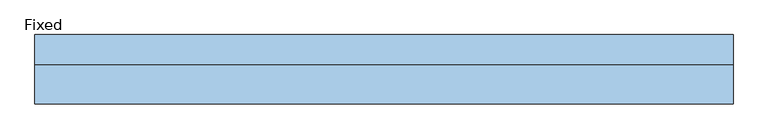
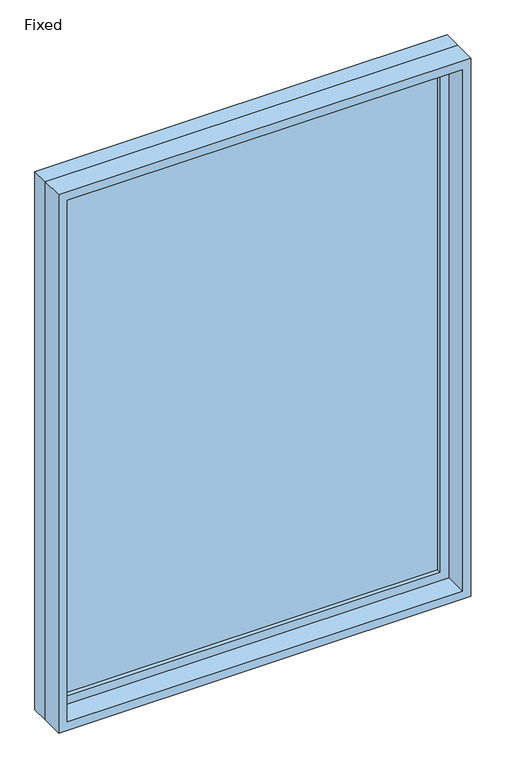
"""IFC4 building model written with IfcOpenShell, lengths in millimetres: window geometry, Fixed."""

from ifc_helpers import new_model, si_unit, frame, origin, place, context, project, spatial, polyline, outline, extrude, source, transform, mapped, element, save


def fixed_17e7873a(model_context):
    return source(origin(), model_context, "Body", "SweptSolid", [
        extrude(outline(polyline([(635.0, 25.4), (-711.2, 25.4), (-711.2, 38.1), (635.0, 38.1), (635.0, 25.4)])), frame((0.0, 0.0, 977.9), z_axis=(0.0, 0.0, 1.0), x_axis=(1.0, 0.0, 0.0)), (0.0, 0.0, 1.0), 1905.0),
        extrude(outline(polyline([(2927.35, -755.65), (933.45, -755.65), (933.45, 679.45), (2927.35, 679.45), (2927.35, -755.65)]), holes=[polyline([(2882.9, -711.2), (2882.9, 635.0), (977.9, 635.0), (977.9, -711.2), (2882.9, -711.2)])]), frame((0.0, 9.525, 0.0), z_axis=(0.0, 1.0, 0.0), x_axis=(0.0, 0.0, 1.0)), (0.0, 0.0, 1.0), 44.45),
        extrude(outline(polyline([(2946.4, -774.7), (914.4, -774.7), (914.4, 698.5), (2946.4, 698.5), (2946.4, -774.7)]), holes=[polyline([(2914.65, -742.95), (2914.65, 666.75), (946.15, 666.75), (946.15, -742.95), (2914.65, -742.95)])]), frame((0.0, -73.025, 0.0), z_axis=(0.0, 1.0, 0.0), x_axis=(0.0, 0.0, 1.0)), (0.0, 0.0, 1.0), 82.55),
        extrude(outline(polyline([(2946.4, 698.5), (2946.4, -774.7), (914.4, -774.7), (914.4, 698.5), (2946.4, 698.5)]), holes=[polyline([(2927.35, 679.45), (933.45, 679.45), (933.45, -755.65), (2927.35, -755.65), (2927.35, 679.45)])]), frame((0.0, 9.525, 0.0), z_axis=(0.0, 1.0, 0.0), x_axis=(0.0, 0.0, 1.0)), (0.0, 0.0, 1.0), 63.5),
    ])


if __name__ == "__main__":
    model = new_model("IFC4")
    model_context = context("Model", 3, world=origin())
    ifc_project = project(units=[si_unit("LENGTHUNIT", "METRE", prefix="MILLI")], contexts=[model_context])
    site = spatial("IfcSite", under=ifc_project)
    building = spatial("IfcBuilding", under=site)
    placement = place(None, origin())
    fixed_shape = fixed_17e7873a(model_context)
    element("IfcWindow", 1, ObjectType="Fixed : 58\"x80\"@11\"", at=placement, inside=building, context=model_context, shape_type="MappedRepresentation", body=[
        mapped(fixed_shape, transform((0.0, 0.0, 0.0), x_axis=(1.0, 0.0, 0.0), y_axis=(0.0, 1.0, 0.0), z_axis=(0.0, 0.0, 1.0))),
    ])
    save(model, "model.ifc")

# Revit data of these elements
# Type "Fixed : 58\"x80\"@11\""
#   Type Mark = "19"
#   Construction Type Id = "GSP4R"
#   Assembly Code = "B2020100"
#   Analytic Construction = "1/8 in Pilkington single glazing"
#   Visual Light Transmittance = 0.9
#   Solar Heat Gain Coefficient = 0.78
#   Heat Transfer Coefficient (U) = 3.6886 W/(m²·K)
#   Height = 6' - 8"
#   Default Sill Height = 3' - 0"
#   Width = 4' - 10"
#   Window Inset = 0' - 0 3/4"
#   Glass Pane Material = Glass
#   Sash Material = Metal Trim
#   Wall Closure = (empty or 0)
# Element 1 (IfcWindow, "Fixed : 58\"x80\"@11\"")
#   Materials on its faces: "Metal Trim", "Glass"
# Materials
#   "Glass": class "Glass", colour RGB 218 227 224, transparency 0.85, Description = "Soda Lime Glass", Cost = 0
#   "Metal Trim": class "Wood", colour RGB 151 137 121, transparency 0, Cost = 0
